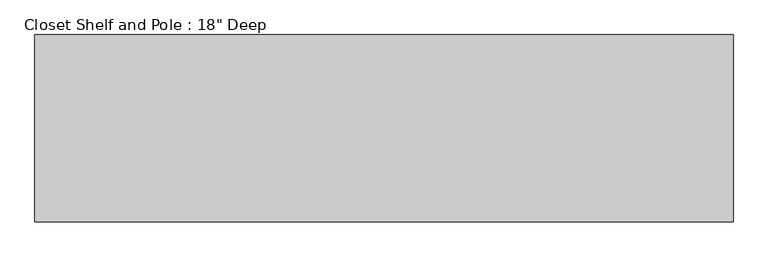
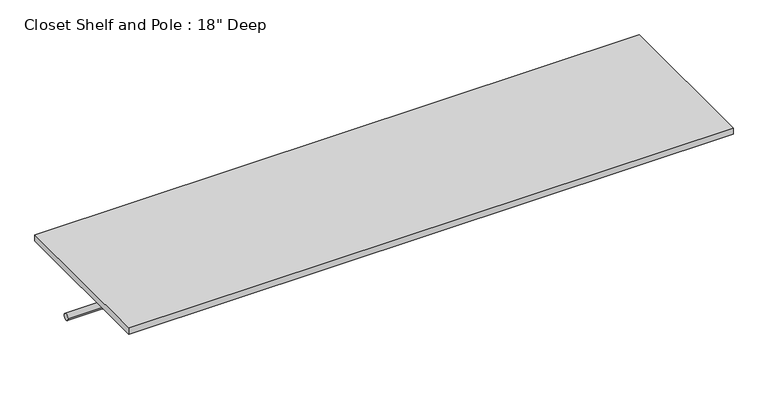
"""IFC4 building model written with IfcOpenShell, lengths in millimetres: proxy geometry."""

from ifc_helpers import new_model, si_unit, point, frame, frame_2d, origin, place, context, project, spatial, polyline, circle_curve, trimmed, segment, composite_curve, outline, extrude, source, transform, mapped, element, save


def proxy_9baf1220(model_context):
    return source(origin(), model_context, "Body", "SweptSolid", [
        extrude(outline(composite_curve([segment(trimmed(circle_curve(frame_2d((304.8, 1676.4)), 9.525), [point((314.325, 1676.4))], [point((295.275, 1676.4))], False, "CARTESIAN"), True, "CONTINUOUS"), segment(trimmed(circle_curve(frame_2d((304.8, 1676.4)), 9.525), [point((295.275, 1676.4))], [point((314.325, 1676.4))], False, "CARTESIAN"), True, "CONTINUOUS")], self_intersect=False)), frame((0.0, 0.0, 0.0), z_axis=(1.0, 0.0, 0.0), x_axis=(0.0, 1.0, 0.0)), (0.0, 0.0, 1.0), 1701.8),
        extrude(outline(polyline([(1701.8, 0.0), (0.0, 0.0), (0.0, 457.2), (1701.8, 457.2), (1701.8, 0.0)])), frame((0.0, 0.0, 1809.75), z_axis=(0.0, 0.0, 1.0), x_axis=(1.0, 0.0, 0.0)), (0.0, 0.0, 1.0), 19.05),
    ])


if __name__ == "__main__":
    model = new_model("IFC4")
    model_context = context("Model", 3, world=origin())
    ifc_project = project(units=[si_unit("LENGTHUNIT", "METRE", prefix="MILLI")], contexts=[model_context])
    site = spatial("IfcSite", under=ifc_project)
    building = spatial("IfcBuilding", under=site)
    placement = place(None, origin())
    proxy_shape = proxy_9baf1220(model_context)
    element("IfcBuildingElementProxy", 1, Name="Closet Shelf and Pole : 18\" Deep", ObjectType="Closet Shelf and Pole : 18\" Deep", at=placement, inside=building, context=model_context, shape_type="MappedRepresentation", body=[
        mapped(proxy_shape, transform((0.0, 0.0, 0.0), x_axis=(1.0, 0.0, 0.0), y_axis=(0.0, 1.0, 0.0), z_axis=(0.0, 0.0, 1.0))),
    ])
    save(model, "model.ifc")

# Revit data of these elements
# Type "Closet Shelf and Pole : 18\" Deep"
#   Shelf Height = 6' - 0"
#   Depth = 1' - 6"
#   built-in parameter 1001306 [instance default] = 4 (stored number, unit not read)
#   Shelf Material = Birch
#   Default Elevation = 0
# Element 1 (IfcBuildingElementProxy, "Closet Shelf and Pole : 18\" Deep")
#   built-in parameter 1001306 = 5.58333 (stored number, unit not read)
#   Materials on its faces: "Birch"
# Materials
#   "Birch": class "Wood", colour RGB 172 132 95, transparency 0, Description = "Betula Alleghaniensis", Cost = 0
